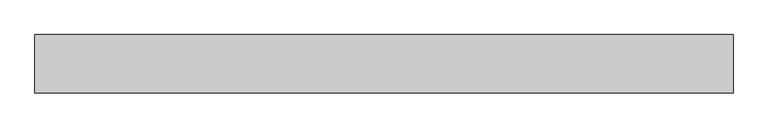
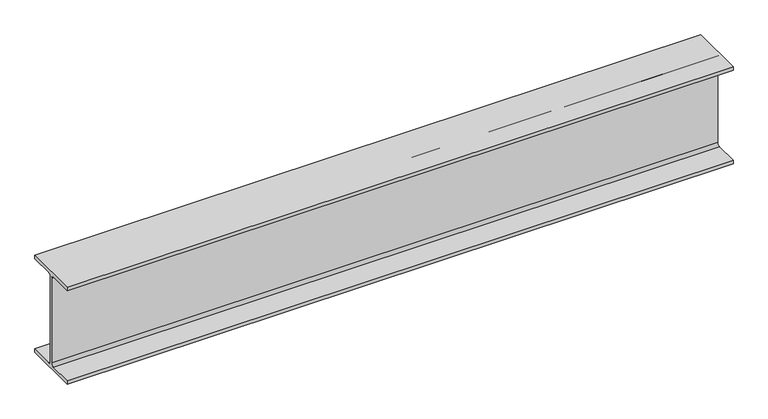
"""IFC4 building model written with IfcOpenShell, lengths in millimetres: beam geometry, Old_Steel Beam_H-KSD3502 : H_SB_ASB_H-194×150x6x9."""

from ifc_helpers import new_model, si_unit, point, frame, frame_2d, origin, place, context, project, spatial, polyline, circle_curve, trimmed, segment, composite_curve, outline, extrude, source, transform, mapped, element, save


def beam_8c5719b2(model_context):
    return source(origin(), model_context, "Body", "SweptSolid", [
        extrude(outline(composite_curve([segment(polyline([(82.5, -141.5), (82.5, -151.7), (-82.5, -151.7), (-82.5, -141.5), (-11.9, -141.5)]), True, "CONTINUOUS"), segment(trimmed(circle_curve(frame_2d((-11.9, -132.6)), 8.9), [point((-11.9, -141.5))], [point((-3.0, -132.6))], True, "CARTESIAN"), True, "CONTINUOUS"), segment(polyline([(-3.0, -132.6), (-3.0, 132.6)]), True, "CONTINUOUS"), segment(trimmed(circle_curve(frame_2d((-11.9, 132.6)), 8.9), [point((-3.0, 132.6))], [point((-11.9, 141.5))], True, "CARTESIAN"), True, "CONTINUOUS"), segment(polyline([(-11.9, 141.5), (-82.5, 141.5), (-82.5, 151.7), (82.5, 151.7), (82.5, 141.5), (11.9, 141.5)]), True, "CONTINUOUS"), segment(trimmed(circle_curve(frame_2d((11.9, 132.6)), 8.9), [point((11.9, 141.5))], [point((3.0, 132.6))], True, "CARTESIAN"), True, "CONTINUOUS"), segment(polyline([(3.0, 132.6), (3.0, -132.6)]), True, "CONTINUOUS"), segment(trimmed(circle_curve(frame_2d((11.9, -132.6)), 8.9), [point((3.0, -132.6))], [point((11.9, -141.5))], True, "CARTESIAN"), True, "CONTINUOUS"), segment(polyline([(11.9, -141.5), (82.5, -141.5)]), True, "CONTINUOUS")], self_intersect=False)), frame((-988.3546085, 0.0, 0.0), z_axis=(1.0, 0.0, 0.0), x_axis=(0.0, 1.0, 0.0)), (0.0, 0.0, 1.0), 1976.709217),
    ])


if __name__ == "__main__":
    model = new_model("IFC4")
    model_context = context("Model", 3, world=origin())
    ifc_project = project(units=[si_unit("LENGTHUNIT", "METRE", prefix="MILLI")], contexts=[model_context])
    site = spatial("IfcSite", under=ifc_project)
    building = spatial("IfcBuilding", under=site)
    placement = place(None, origin())
    beam_shape = beam_8c5719b2(model_context)
    element("IfcBeam", 1, ObjectType="Old_Steel Beam_H-KSD3502 : H_SB_ASB_H-194×150x6x9", at=placement, inside=building, context=model_context, shape_type="MappedRepresentation", body=[
        mapped(beam_shape, transform((0.0, 0.0, 0.0), x_axis=(1.0, 0.0, 0.0), y_axis=(0.0, 1.0, 0.0), z_axis=(0.0, 0.0, 1.0))),
    ])
    save(model, "model.ifc")

# Revit data of these elements
# Type "Old_Steel Beam_H-KSD3502 : H_SB_ASB_H-194×150x6x9"
#   Width = 15.0 cm
#   Web Thickness = 0.6 cm
#   Web Fillet = 1.3 cm
#   Warping Constant = 43316.0 cm⁶
#   Torsional Moment of Inertia = 8.622 cm⁴
#   Torsional Modulus = 1.0 cm³
#   Section Area = 39.01 cm²
#   Plastic Modulus weak axis = 104.0 cm³
#   Plastic Modulus strong axis = 309.0 cm³
#   Perimeter = 0.95 m²/m
#   Nominal Weight = 30.60 kgf/m
#   Moment of Inertia weak axis = 507.00 cm⁴
#   Moment of Inertia strong axis = 2690.00 cm⁴
#   Height = 19.4 cm
#   Flange Thickness = 0.9 cm
#   Elastic Modulus weak axis = 67.6 cm³
#   Elastic Modulus strong axis = 277.0 cm³
#   Centroid Vertical = 9.7 cm
#   Centroid Horizontal = 7.5 cm
#   Length [instance default] = 1.5240 m
#   Structural Material [instance default] = Steel, 45-345
#   Assembly Code = ""
# Element 1 (IfcBeam, "Old_Steel Beam_H-KSD3502 : H_SB_ASB_H-194×150x6x9")
#   Structural Material = none
# Materials
#   "Steel, 45-345": class "Metal", colour RGB 189 187 185, transparency 0, Description = "Steel 345 MPa", Cost = 0
